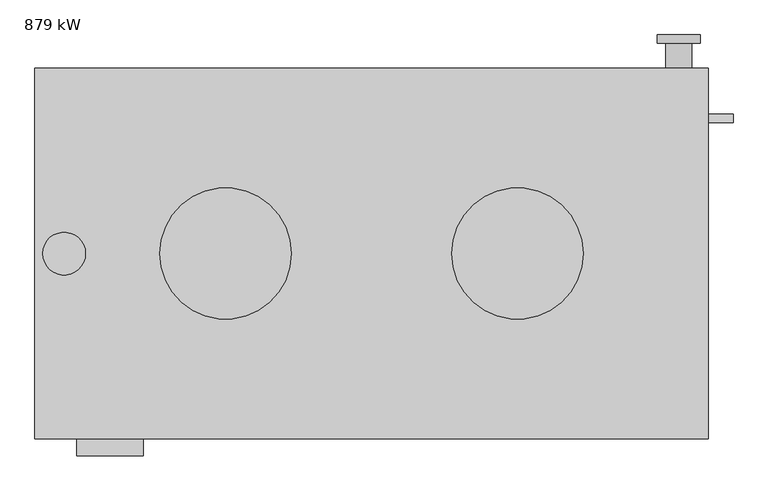
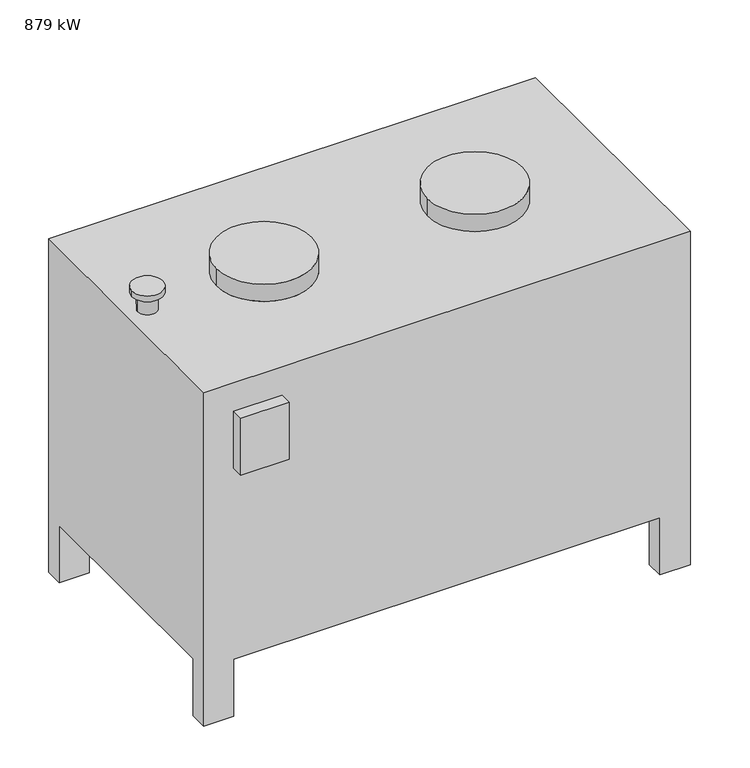
"""IFC4 building model written with IfcOpenShell, lengths in millimetres: proxy geometry, M_Watertube Boiler - 879-6153 kW : 879 kW."""

import ifcopenshell
import ifcopenshell.guid

model = None  # the IFC model being written
_history = None  # IfcOwnerHistory: only IFC2X3 demands one
_inside = {}  # id of a spatial element -> (the spatial element, [elements in it])
_under = {}  # id of a project, library or spatial element -> (it, [spatial elements below it])
_declared = {}  # id of a project -> (the project, [libraries it declares])
_typed = {}  # id of a type object -> (the type object, [elements of that type])
_made_of = {}  # id of a material, layer set ... -> (it, [elements and type objects made of it])


def new_model(schema):
    """Start an empty IFC model of exactly this schema.

    Asked for "IFC4X3", IfcOpenShell would pick the latest addendum, in which some entities
    have other attributes; the version numbers below select the first issue.
    IFC2X3 requires an IfcOwnerHistory on every rooted entity: one is made here for all.
    """
    global model, _history
    if schema == "IFC4X3":
        model = ifcopenshell.file(schema_version=(4, 3, 0, 0))
    else:
        model = ifcopenshell.file(schema=schema)
    _inside.clear()
    _under.clear()
    _declared.clear()
    _typed.clear()
    _made_of.clear()
    _history = None
    if model.schema == "IFC2X3":
        org = make("IfcOrganization", Name="unknown")
        user = make(
            "IfcPersonAndOrganization",
            ThePerson=make("IfcPerson", FamilyName="unknown"),
            TheOrganization=org,
        )
        app = make(
            "IfcApplication",
            ApplicationDeveloper=org,
            Version="unknown",
            ApplicationFullName="unknown",
            ApplicationIdentifier="unknown",
        )
        _history = make(
            "IfcOwnerHistory",
            OwningUser=user,
            OwningApplication=app,
            ChangeAction="ADDED",
            CreationDate=0,
        )
    return model


def make(cls, **values):
    """One entity of the class cls with the attributes given. An attribute that is None is left unset."""
    return model.create_entity(
        cls, **{name: value for name, value in values.items() if value is not None}
    )


def rooted(cls, **values):
    """An entity with a GlobalId (a new one), such as an element, a storey or a relation."""
    return make(cls, GlobalId=ifcopenshell.guid.new(), OwnerHistory=_history, **values)


def si_unit(unit_type, name, prefix=None):
    """IfcSIUnit, for example si_unit("LENGTHUNIT", "METRE", prefix="MILLI")."""
    return make("IfcSIUnit", UnitType=unit_type, Prefix=prefix, Name=name)


def assignment(units):
    """IfcUnitAssignment: the units of a project."""
    return None if units is None else make("IfcUnitAssignment", Units=units)


def point(xyz):
    """IfcCartesianPoint."""
    return None if xyz is None else make("IfcCartesianPoint", Coordinates=xyz)


def direction(xyz):
    """IfcDirection."""
    return None if xyz is None else make("IfcDirection", DirectionRatios=xyz)


def frame(location, z_axis=None, x_axis=None):
    """IfcAxis2Placement3D, a coordinate frame: its origin and axes. An axis left out is left unset."""
    return make(
        "IfcAxis2Placement3D",
        Location=point(location),
        Axis=direction(z_axis),
        RefDirection=direction(x_axis),
    )


def frame_2d(location, x_axis=None):
    """IfcAxis2Placement2D, a coordinate frame in the plane: its origin and x axis."""
    return make(
        "IfcAxis2Placement2D", Location=point(location), RefDirection=direction(x_axis)
    )


def origin():
    """The frame at (0, 0, 0) with its axes left unset."""
    return frame((0.0, 0.0, 0.0))


def place(relative_to, where):
    """IfcLocalPlacement: puts the frame where relative to a parent placement (None: the world)."""
    return make(
        "IfcLocalPlacement", PlacementRelTo=relative_to, RelativePlacement=where
    )


def context(
    kind, dimensions, precision=None, world=None, true_north=None, identifier=None
):
    """IfcGeometricRepresentationContext, for example the 3D "Model" context."""
    return make(
        "IfcGeometricRepresentationContext",
        ContextIdentifier=identifier,
        ContextType=kind,
        CoordinateSpaceDimension=dimensions,
        Precision=precision,
        WorldCoordinateSystem=world,
        TrueNorth=true_north,
    )


def project(units=None, contexts=None):
    """IfcProject with its units and contexts."""
    return rooted(
        "IfcProject",
        Name="project",
        RepresentationContexts=contexts,
        UnitsInContext=assignment(units),
    )


def spatial(cls, under=None, at=None, **own):
    """A site, building, storey or space (cls), placed at a placement, below another one or the project."""
    s = rooted(cls, ObjectPlacement=at, **own)
    if under is not None:
        _under.setdefault(under.id(), (under, []))[1].append(s)
    return s


def circle_curve(where, radius):
    """IfcCircle in the frame where."""
    return make("IfcCircle", Position=where, Radius=radius)


def trimmed(basis, trim1, trim2, sense, master):
    """IfcTrimmedCurve: the piece of a basis curve between two trims."""
    return make(
        "IfcTrimmedCurve",
        BasisCurve=basis,
        Trim1=trim1,
        Trim2=trim2,
        SenseAgreement=sense,
        MasterRepresentation=master,
    )


def segment(curve, same_sense, transition):
    """IfcCompositeCurveSegment."""
    return make(
        "IfcCompositeCurveSegment",
        Transition=transition,
        SameSense=same_sense,
        ParentCurve=curve,
    )


def composite_curve(segments, self_intersect=None):
    """IfcCompositeCurve: segments joined end to end."""
    return make("IfcCompositeCurve", Segments=segments, SelfIntersect=self_intersect)


def outline(outer, holes=None, kind="AREA"):
    """IfcArbitraryClosedProfileDef: a profile drawn as a closed curve; with holes, ...WithVoids."""
    if holes is None:
        return make("IfcArbitraryClosedProfileDef", ProfileType=kind, OuterCurve=outer)
    return make(
        "IfcArbitraryProfileDefWithVoids",
        ProfileType=kind,
        OuterCurve=outer,
        InnerCurves=holes,
    )


def extrude(swept, where, along, depth):
    """IfcExtrudedAreaSolid: the profile swept, set in the frame where, extruded along a direction by depth."""
    return make(
        "IfcExtrudedAreaSolid",
        SweptArea=swept,
        Position=where,
        ExtrudedDirection=direction(along),
        Depth=depth,
    )


def shape(context_of_items, identifier, shape_type, items):
    """IfcShapeRepresentation: the items that make up one representation, for example the "Body"."""
    return make(
        "IfcShapeRepresentation",
        ContextOfItems=context_of_items,
        RepresentationIdentifier=identifier,
        RepresentationType=shape_type,
        Items=items,
    )


def source(mapping_origin, context_of_items, identifier, shape_type, items):
    """IfcRepresentationMap: a shape defined once, which mapped items show again and again."""
    return make(
        "IfcRepresentationMap",
        MappingOrigin=mapping_origin,
        MappedRepresentation=shape(context_of_items, identifier, shape_type, items),
    )


def transform(
    local_origin,
    x_axis=None,
    y_axis=None,
    z_axis=None,
    scale=None,
    scale2=None,
    scale3=None,
    uniform=True,
):
    """IfcCartesianTransformationOperator3D, or its non-uniform kind. x_axis, y_axis, z_axis: its Axis1, 2, 3."""
    if uniform:
        return make(
            "IfcCartesianTransformationOperator3D",
            Axis1=direction(x_axis),
            Axis2=direction(y_axis),
            LocalOrigin=point(local_origin),
            Scale=scale,
            Axis3=direction(z_axis),
        )
    return make(
        "IfcCartesianTransformationOperator3DnonUniform",
        Axis1=direction(x_axis),
        Axis2=direction(y_axis),
        LocalOrigin=point(local_origin),
        Scale=scale,
        Axis3=direction(z_axis),
        Scale2=scale2,
        Scale3=scale3,
    )


def mapped(mapping_source, mapping_target):
    """IfcMappedItem: shows the shape of a source again, moved by a transform."""
    return make(
        "IfcMappedItem", MappingSource=mapping_source, MappingTarget=mapping_target
    )


def made_of(thing, what):
    """Note that an element or type object is made of a material, layer set ...; save() writes the relation."""
    if what is not None:
        _made_of.setdefault(what.id(), (what, []))[1].append(thing)
    return thing


def element(
    cls,
    number,
    at=None,
    inside=None,
    cuts=None,
    type_object=None,
    material=None,
    context=None,
    identifier="Body",
    shape_type=None,
    held_by="IfcProductDefinitionShape",
    body=None,
    shapes=None,
    **own,
):
    """One element of the class cls, such as IfcWall. Its Tag is "e" and its number.

    at: its placement. inside: the storey or other place that contains it. cuts: it is an
    opening in that element (IfcRelVoidsElement). A single representation is given by context,
    identifier, shape_type and body (its items); several are given by shapes. held_by: the class
    of the entity that holds the representations. save() writes the other relations.
    """
    e = rooted(cls, Tag="e%d" % number, ObjectPlacement=at, **own)
    if body is not None:
        shapes = [shape(context, identifier, shape_type, body)]
    if shapes is not None:
        e.Representation = make(held_by, Representations=shapes)
    if inside is not None:
        _inside.setdefault(inside.id(), (inside, []))[1].append(e)
    if cuts is not None:
        rooted(
            "IfcRelVoidsElement", RelatingBuildingElement=cuts, RelatedOpeningElement=e
        )
    if type_object is not None:
        _typed.setdefault(type_object.id(), (type_object, []))[1].append(e)
    return made_of(e, material)


def aggregate(whole, parts):
    """IfcRelAggregates: a whole, such as a stair, and the parts it consists of."""
    return rooted("IfcRelAggregates", RelatingObject=whole, RelatedObjects=parts)


def save(model, path):
    """Write the relations noted so far, then the file.

    IfcRelAggregates (storeys below a building ...), IfcRelContainedInSpatialStructure (elements
    in a storey), IfcRelDefinesByType, IfcRelAssociatesMaterial and IfcRelDeclares: one each for
    every whole, place, type object, material and project.
    """
    for whole, parts in _under.values():
        aggregate(whole, parts)
    for where, things in _inside.values():
        rooted(
            "IfcRelContainedInSpatialStructure",
            RelatedElements=things,
            RelatingStructure=where,
        )
    for kind, things in _typed.values():
        rooted("IfcRelDefinesByType", RelatedObjects=things, RelatingType=kind)
    for what, things in _made_of.values():
        rooted("IfcRelAssociatesMaterial", RelatedObjects=things, RelatingMaterial=what)
    for by, libraries in _declared.values():
        rooted("IfcRelDeclares", RelatingContext=by, RelatedDefinitions=libraries)
    model.write(path)


def plane_surface(at):
    """IfcPlane: the flat surface through the origin of the frame at, square to its z axis."""
    return make("IfcPlane", Position=at)


def cylinder_surface(at, radius):
    """IfcCylindricalSurface: all points at the distance radius from the z axis of the frame at."""
    return make("IfcCylindricalSurface", Position=at, Radius=radius)


def advanced_brep(points, edges, surfaces, faces):
    """IfcAdvancedBrep: a solid bounded by faces that lie on surfaces and meet in shared edges.

    An edge is (start, end): straight between two places in points (the first is 0);
    or (start, end, curve); or (start, end, curve, False) where it runs against its curve.
    A face is (place in surfaces, loops), or (place, loops, False) where it looks against
    its surface's normal. A loop lists edges by number (the first is 1), with a minus sign
    where the edge is run from its end to its start. The first loop is the outer one.
    """
    corners = [point(p) for p in points]
    vertices = [make("IfcVertexPoint", VertexGeometry=c) for c in corners]
    made = []
    for start, end, *more in edges:
        made.append(
            make(
                "IfcEdgeCurve",
                EdgeStart=vertices[start],
                EdgeEnd=vertices[end],
                EdgeGeometry=more[0] if more else make("IfcPolyline", Points=[corners[start], corners[end]]),
                SameSense=more[1] if len(more) > 1 else True,
            )
        )
    hull = []
    for where, loops, *sense in faces:
        bounds = []
        for j, loop in enumerate(loops):
            ring = [make("IfcOrientedEdge", EdgeElement=made[abs(k) - 1], Orientation=k > 0) for k in loop]
            bounds.append(
                make(
                    "IfcFaceOuterBound" if j == 0 else "IfcFaceBound",
                    Bound=make("IfcEdgeLoop", EdgeList=ring),
                    Orientation=True,
                )
            )
        hull.append(make("IfcAdvancedFace", Bounds=bounds, FaceSurface=surfaces[where], SameSense=sense[0] if sense else True))
    return make("IfcAdvancedBrep", Outer=make("IfcClosedShell", CfsFaces=hull))


def proxy_879_kw_a7649213(model_context):
    return source(origin(), model_context, "Body", "SolidModel", [
        extrude(outline(composite_curve([segment(trimmed(circle_curve(frame_2d((826.0, 1961.0)), 40.0), [point((826.0, 1921.0))], [point((826.0, 2001.0))], False, "CARTESIAN"), True, "CONTINUOUS"), segment(trimmed(circle_curve(frame_2d((826.0, 1961.0)), 40.0), [point((826.0, 2001.0))], [point((826.0, 1921.0))], False, "CARTESIAN"), True, "CONTINUOUS")], self_intersect=False)), frame((0.0, 1130.0, 0.0), z_axis=(0.0, 1.0, 0.0), x_axis=(0.0, 0.0, 1.0)), (0.0, 0.0, 1.0), 76.2),
        extrude(outline(composite_curve([segment(trimmed(circle_curve(frame_2d((826.0, 1961.0)), 65.0), [point((826.0, 1896.0))], [point((826.0, 2026.0))], False, "CARTESIAN"), True, "CONTINUOUS"), segment(trimmed(circle_curve(frame_2d((826.0, 1961.0)), 65.0), [point((826.0, 2026.0))], [point((826.0, 1896.0))], False, "CARTESIAN"), True, "CONTINUOUS")], self_intersect=False)), frame((0.0, 1206.5, 0.0), z_axis=(0.0, 1.0, 0.0), x_axis=(0.0, 0.0, 1.0)), (0.0, 0.0, 1.0), 25.1),
        extrude(outline(composite_curve([segment(trimmed(circle_curve(frame_2d((977.6, 508.0)), 12.7), [point((964.9, 508.0))], [point((990.3, 508.0))], False, "CARTESIAN"), True, "CONTINUOUS"), segment(trimmed(circle_curve(frame_2d((977.6, 508.0)), 12.7), [point((990.3, 508.0))], [point((964.9, 508.0))], False, "CARTESIAN"), True, "CONTINUOUS")], self_intersect=False)), frame((2050.0, 0.0, 0.0), z_axis=(1.0, 0.0, 0.0), x_axis=(0.0, 1.0, 0.0)), (0.0, 0.0, 1.0), 76.2),
        extrude(outline(composite_curve([segment(trimmed(circle_curve(frame_2d((1796.0, 203.2)), 25.0), [point((1771.0, 203.2))], [point((1821.0, 203.2))], False, "CARTESIAN"), True, "CONTINUOUS"), segment(trimmed(circle_curve(frame_2d((1796.0, 203.2)), 25.0), [point((1821.0, 203.2))], [point((1771.0, 203.2))], False, "CARTESIAN"), True, "CONTINUOUS")], self_intersect=False)), frame((0.0, 0.0, 177.8), z_axis=(0.0, 0.0, 1.0), x_axis=(1.0, 0.0, 0.0)), (0.0, 0.0, 1.0), 76.2),
        advanced_brep(
        [(1923.0, 0.0, 254.0), (1923.0, 0.0, 0.0), (2050.0, 0.0, 0.0), (2050.0, 0.0, 1485.0), (0.0, 0.0, 1485.0), (0.0, 0.0, 0.0), (127.0, 0.0, 0.0), (127.0, 0.0, 254.0), (127.0, 0.0, 1358.0), (330.2, 0.0, 1358.0), (330.2, 0.0, 1104.0), (127.0, 0.0, 1104.0), (2050.0, 76.2, 254.0), (2050.0, 76.2, 0.0), (1923.0, 76.2, 0.0), (1923.0, 76.2, 254.0), (2050.0, 1053.8, 254.0), (2050.0, 1053.8, 0.0), (2050.0, 1130.0, 0.0), (2050.0, 1130.0, 1485.0), (1923.0, 1053.8, 254.0), (1923.0, 1053.8, 0.0), (1923.0, 1130.0, 0.0), (1923.0, 1130.0, 254.0), (127.0, 1130.0, 254.0), (127.0, 1130.0, 0.0), (0.0, 1130.0, 0.0), (0.0, 1130.0, 1485.0), (129.0, 565.0, 1485.0), (49.0, 565.0, 1485.0), (780.5, 565.0, 1485.0), (380.5, 565.0, 1485.0), (1669.5, 565.0, 1485.0), (1269.5, 565.0, 1485.0), (127.0, 76.2, 254.0), (0.0, 76.2, 254.0), (0.0, 1053.8, 254.0), (127.0, 1053.8, 254.0), (0.0, 1053.8, 0.0), (0.0, 76.2, 0.0), (49.0, 565.0, 1561.2), (129.0, 565.0, 1561.2), (24.0, 565.0, 1586.6), (154.0, 565.0, 1586.6), (24.0, 565.0, 1561.2), (154.0, 565.0, 1561.2), (380.5, 565.0, 1561.2), (780.5, 565.0, 1561.2), (1269.5, 565.0, 1561.2), (1669.5, 565.0, 1561.2), (330.2, -50.8, 1358.0), (127.0, -50.8, 1358.0), (127.0, -50.8, 1104.0), (330.2, -50.8, 1104.0), (127.0, 76.2, 0.0), (127.0, 1053.8, 0.0)],
        [
            (0, 1),
            (1, 2),
            (2, 3),
            (3, 4),
            (4, 5),
            (5, 6),
            (6, 7),
            (7, 0),
            (8, 9),
            (9, 10),
            (10, 11),
            (11, 8),
            (12, 13),
            (13, 14),
            (14, 15),
            (15, 12),
            (0, 15),
            (14, 1),
            (13, 2),
            (12, 16),
            (16, 17),
            (17, 18),
            (18, 19),
            (19, 3),
            (20, 21),
            (21, 17),
            (16, 20),
            (18, 22),
            (22, 23),
            (23, 24),
            (24, 25),
            (25, 26),
            (26, 27),
            (27, 19),
            (20, 23),
            (22, 21),
            (27, 4),
            (28, 29, circle_curve(frame((89.0, 565.0, 1485.0), z_axis=(0.0, 0.0, -1.0), x_axis=(1.0, 0.0, 0.0)), 40.0)),
            (29, 28, circle_curve(frame((89.0, 565.0, 1485.0), z_axis=(0.0, 0.0, -1.0), x_axis=(1.0, 0.0, 0.0)), 40.0)),
            (30, 31, circle_curve(frame((580.5, 565.0, 1485.0), z_axis=(0.0, 0.0, -1.0), x_axis=(1.0, 0.0, 0.0)), 200.0)),
            (31, 30, circle_curve(frame((580.5, 565.0, 1485.0), z_axis=(0.0, 0.0, -1.0), x_axis=(1.0, 0.0, 0.0)), 200.0)),
            (32, 33, circle_curve(frame((1469.5, 565.0, 1485.0), z_axis=(0.0, 0.0, -1.0), x_axis=(1.0, 0.0, 0.0)), 200.0)),
            (33, 32, circle_curve(frame((1469.5, 565.0, 1485.0), z_axis=(0.0, 0.0, -1.0), x_axis=(1.0, 0.0, 0.0)), 200.0)),
            (7, 34),
            (34, 35),
            (35, 36),
            (36, 37),
            (37, 24),
            (26, 38),
            (38, 36),
            (35, 39),
            (39, 5),
            (40, 29),
            (28, 41),
            (41, 40, circle_curve(frame((89.0, 565.0, 1561.2), z_axis=(0.0, 0.0, -1.0), x_axis=(1.0, 0.0, 0.0)), 40.0)),
            (40, 41, circle_curve(frame((89.0, 565.0, 1561.2), z_axis=(0.0, 0.0, -1.0), x_axis=(1.0, 0.0, 0.0)), 40.0)),
            (42, 43, circle_curve(frame((89.0, 565.0, 1586.6), z_axis=(0.0, 0.0, 1.0), x_axis=(1.0, 0.0, 0.0)), 65.0)),
            (43, 42, circle_curve(frame((89.0, 565.0, 1586.6), z_axis=(0.0, 0.0, 1.0), x_axis=(1.0, 0.0, 0.0)), 65.0)),
            (44, 45, circle_curve(frame((89.0, 565.0, 1561.2), z_axis=(0.0, 0.0, -1.0), x_axis=(1.0, 0.0, 0.0)), 65.0)),
            (45, 44, circle_curve(frame((89.0, 565.0, 1561.2), z_axis=(0.0, 0.0, -1.0), x_axis=(1.0, 0.0, 0.0)), 65.0)),
            (42, 44),
            (45, 43),
            (46, 47, circle_curve(frame((580.5, 565.0, 1561.2), z_axis=(0.0, 0.0, 1.0), x_axis=(1.0, 0.0, 0.0)), 200.0)),
            (47, 46, circle_curve(frame((580.5, 565.0, 1561.2), z_axis=(0.0, 0.0, 1.0), x_axis=(1.0, 0.0, 0.0)), 200.0)),
            (48, 49, circle_curve(frame((1469.5, 565.0, 1561.2), z_axis=(0.0, 0.0, 1.0), x_axis=(1.0, 0.0, 0.0)), 200.0)),
            (49, 48, circle_curve(frame((1469.5, 565.0, 1561.2), z_axis=(0.0, 0.0, 1.0), x_axis=(1.0, 0.0, 0.0)), 200.0)),
            (46, 31),
            (30, 47),
            (48, 33),
            (32, 49),
            (50, 51),
            (51, 52),
            (52, 53),
            (53, 50),
            (50, 9),
            (8, 51),
            (11, 52),
            (10, 53),
            (34, 54),
            (54, 39),
            (54, 6),
            (38, 55),
            (55, 37),
            (25, 55),
        ],
        [
            plane_surface(frame((1923.0, 0.0, 254.0), z_axis=(0.0, -1.0, 0.0), x_axis=(0.0, 0.0, -1.0))),
            plane_surface(frame((1923.0, 76.2, 254.0), z_axis=(0.0, 1.0, 0.0), x_axis=(0.0, 0.0, 1.0))),
            plane_surface(frame((1923.0, 0.0, 254.0), z_axis=(-1.0, 0.0, 0.0), x_axis=(0.0, 1.0, 0.0))),
            plane_surface(frame((1923.0, 0.0, 0.0), z_axis=(0.0, 0.0, -1.0), x_axis=(0.0, 1.0, 0.0))),
            plane_surface(frame((2050.0, 0.0, 0.0), z_axis=(1.0, 0.0, 0.0), x_axis=(0.0, 1.0, 0.0))),
            plane_surface(frame((1923.0, 1053.8, 254.0), z_axis=(0.0, -1.0, 0.0), x_axis=(0.0, 0.0, -1.0))),
            plane_surface(frame((1923.0, 1130.0, 254.0), z_axis=(0.0, 1.0, 0.0), x_axis=(0.0, 0.0, 1.0))),
            plane_surface(frame((1923.0, 1053.8, 254.0), z_axis=(-1.0, 0.0, 0.0), x_axis=(0.0, 1.0, 0.0))),
            plane_surface(frame((1923.0, 1053.8, 0.0), z_axis=(0.0, 0.0, -1.0), x_axis=(0.0, 1.0, 0.0))),
            plane_surface(frame((0.0, 1130.0, 1485.0), z_axis=(0.0, 0.0, 1.0), x_axis=(-1.0, 0.0, 0.0))),
            plane_surface(frame((0.0, 1130.0, 254.0), z_axis=(0.0, 0.0, -1.0), x_axis=(1.0, 0.0, 0.0))),
            plane_surface(frame((0.0, 1130.0, 1485.0), z_axis=(-1.0, 0.0, 0.0), x_axis=(0.0, 0.0, -1.0))),
            cylinder_surface(frame((89.0, 565.0, 1485.0), z_axis=(0.0, 0.0, 1.0), x_axis=(1.0, 0.0, 0.0)), 40.0),
            plane_surface(frame((154.0, 565.0, 1586.6), z_axis=(0.0, 0.0, 1.0), x_axis=(0.0, 1.0, 0.0))),
            plane_surface(frame((154.0, 565.0, 1561.2), z_axis=(0.0, 0.0, -1.0), x_axis=(0.0, -1.0, 0.0))),
            cylinder_surface(frame((89.0, 565.0, 1561.2), z_axis=(0.0, 0.0, 1.0), x_axis=(1.0, 0.0, 0.0)), 65.0),
            plane_surface(frame((780.5, 565.0, 1561.2), z_axis=(0.0, 0.0, 1.0), x_axis=(0.0, 1.0, 0.0))),
            cylinder_surface(frame((580.5, 565.0, 1485.0), z_axis=(0.0, 0.0, 1.0), x_axis=(1.0, 0.0, 0.0)), 200.0),
            cylinder_surface(frame((1469.5, 565.0, 0.0), z_axis=(0.0, 0.0, 1.0), x_axis=(1.0, 0.0, 0.0)), 200.0),
            plane_surface(frame((127.0, -50.8, 1358.0), z_axis=(0.0, -1.0, 0.0), x_axis=(-1.0, 0.0, 0.0))),
            plane_surface(frame((330.2, -50.8, 1358.0), z_axis=(0.0, 0.0, 1.0), x_axis=(0.0, 1.0, 0.0))),
            plane_surface(frame((127.0, -50.8, 1358.0), z_axis=(-1.0, 0.0, 0.0), x_axis=(0.0, 1.0, 0.0))),
            plane_surface(frame((127.0, -50.8, 1104.0), z_axis=(0.0, 0.0, -1.0), x_axis=(0.0, 1.0, 0.0))),
            plane_surface(frame((330.2, -50.8, 1104.0), z_axis=(1.0, 0.0, 0.0), x_axis=(0.0, 1.0, 0.0))),
            plane_surface(frame((127.0, 76.2, 0.0), z_axis=(0.0, 1.0, 0.0), x_axis=(-1.0, 0.0, 0.0))),
            plane_surface(frame((0.0, 0.0, 0.0), z_axis=(0.0, 0.0, -1.0), x_axis=(0.0, 1.0, 0.0))),
            plane_surface(frame((127.0, 0.0, 0.0), z_axis=(1.0, 0.0, 0.0), x_axis=(0.0, 1.0, 0.0))),
            plane_surface(frame((0.0, 1053.8, 173.9475615), z_axis=(0.0, -1.0, 0.0), x_axis=(0.0, 0.0, -1.0))),
            plane_surface(frame((0.0, 1053.8, 0.0), z_axis=(0.0, 0.0, -1.0), x_axis=(0.0, 1.0, 0.0))),
            plane_surface(frame((127.0, 1053.8, 0.0), z_axis=(1.0, 0.0, 0.0), x_axis=(0.0, 1.0, 0.0))),
        ],
        [
            (0, [[1, 2, 3, 4, 5, 6, 7, 8], [9, 10, 11, 12]]),
            (1, [[13, 14, 15, 16]]),
            (2, [[-1, 17, -15, 18]]),
            (3, [[-2, -18, -14, 19]]),
            (4, [[-13, 20, 21, 22, 23, 24, -3, -19]]),
            (5, [[25, 26, -21, 27]]),
            (6, [[28, 29, 30, 31, 32, 33, 34, -23]]),
            (7, [[-25, 35, -29, 36]]),
            (8, [[-26, -36, -28, -22]]),
            (9, [[-34, 37, -4, -24], [38, 39], [40, 41], [42, 43]]),
            (10, [[-20, -16, -17, -8, 44, 45, 46, 47, 48, -30, -35, -27]]),
            (11, [[-37, -33, 49, 50, -46, 51, 52, -5]]),
            (12, [[53, -38, 54, 55]]),
            (12, [[-53, 56, -54, -39]]),
            (13, [[57, 58]]),
            (14, [[59, 60], [-55, -56]]),
            (15, [[-57, 61, -60, 62]]),
            (15, [[-58, -62, -59, -61]]),
            (16, [[63, 64]]),
            (16, [[65, 66]]),
            (17, [[-63, 67, -40, 68]]),
            (17, [[-64, -68, -41, -67]]),
            (18, [[-65, 69, -42, 70]]),
            (18, [[-66, -70, -43, -69]]),
            (19, [[71, 72, 73, 74]]),
            (20, [[-71, 75, -9, 76]]),
            (21, [[-72, -76, -12, 77]]),
            (22, [[-73, -77, -11, 78]]),
            (23, [[-74, -78, -10, -75]]),
            (24, [[-51, -45, 79, 80]]),
            (25, [[-6, -52, -80, 81]]),
            (26, [[-7, -81, -79, -44]]),
            (27, [[-50, 82, 83, -47]]),
            (28, [[-82, -49, -32, 84]]),
            (29, [[-83, -84, -31, -48]]),
        ],
    ),
        extrude(outline(composite_curve([segment(trimmed(circle_curve(frame_2d((977.6, 508.0)), 12.7), [point((964.9, 508.0))], [point((990.3, 508.0))], False, "CARTESIAN"), True, "CONTINUOUS"), segment(trimmed(circle_curve(frame_2d((977.6, 508.0)), 12.7), [point((990.3, 508.0))], [point((964.9, 508.0))], False, "CARTESIAN"), True, "CONTINUOUS")], self_intersect=False)), frame((2050.0, 0.0, 0.0), z_axis=(1.0, 0.0, 0.0), x_axis=(0.0, 1.0, 0.0)), (0.0, 0.0, 1.0), 76.2),
        extrude(outline(composite_curve([segment(trimmed(circle_curve(frame_2d((826.0, 1961.0)), 40.0), [point((826.0, 1921.0))], [point((826.0, 2001.0))], False, "CARTESIAN"), True, "CONTINUOUS"), segment(trimmed(circle_curve(frame_2d((826.0, 1961.0)), 40.0), [point((826.0, 2001.0))], [point((826.0, 1921.0))], False, "CARTESIAN"), True, "CONTINUOUS")], self_intersect=False)), frame((0.0, 1130.0, 0.0), z_axis=(0.0, 1.0, 0.0), x_axis=(0.0, 0.0, 1.0)), (0.0, 0.0, 1.0), 76.2),
        extrude(outline(composite_curve([segment(trimmed(circle_curve(frame_2d((826.0, 1961.0)), 65.0), [point((826.0, 1896.0))], [point((826.0, 2026.0))], False, "CARTESIAN"), True, "CONTINUOUS"), segment(trimmed(circle_curve(frame_2d((826.0, 1961.0)), 65.0), [point((826.0, 2026.0))], [point((826.0, 1896.0))], False, "CARTESIAN"), True, "CONTINUOUS")], self_intersect=False)), frame((0.0, 1206.2, 0.0), z_axis=(0.0, 1.0, 0.0), x_axis=(0.0, 0.0, 1.0)), (0.0, 0.0, 1.0), 25.4),
    ])


if __name__ == "__main__":
    model = new_model("IFC4")
    model_context = context("Model", 3, world=origin())
    ifc_project = project(units=[si_unit("LENGTHUNIT", "METRE", prefix="MILLI")], contexts=[model_context])
    site = spatial("IfcSite", under=ifc_project)
    building = spatial("IfcBuilding", under=site)
    placement = place(None, origin())
    proxy_879_kw_shape = proxy_879_kw_a7649213(model_context)
    element("IfcBuildingElementProxy", 1, Name="M_Watertube Boiler - 879-6153 kW : 879 kW", ObjectType="M_Watertube Boiler - 879-6153 kW : 879 kW", at=placement, inside=building, context=model_context, shape_type="MappedRepresentation", body=[
        mapped(proxy_879_kw_shape, transform((0.0, 0.0, 0.0), x_axis=(1.0, 0.0, 0.0), y_axis=(0.0, 1.0, 0.0), z_axis=(0.0, 0.0, 1.0))),
    ])
    save(model, "model.ifc")

# Revit data of these elements
# Type "M_Watertube Boiler - 879-6153 kW : 879 kW"
#   Model = "096967565434gdewtg"
#   Manufacturer = "Boilers Inc"
#   Description = "Boiler"
#   COBie.Type.CreatedBy = "design@eagle.com"
#   COBie.Type.CreatedOn = "2016-09-13T05:47:35"
#   COBie.Type.Name = "Mechanical Equipment_M_Watertube Boiler - 879-6153 kW_879 kW"
#   COBie.Type.Category = "23-75 10 11 14 34 : Steel Water-Tube Boilers"
#   COBie.Type.Description = "Boiler"
#   COBie.Type.Manufacturer = "Boilers Inc"
#   COBie.Type.ModelNumber = "096967565434gdewtg"
#   COBie.Type.ReplacementCost = 0
#   Water Volume [instance default] = 4.22 m³
#   Water Pressure Drop [instance default] = 11700.0 Pa
#   Water Flow [instance default] = 15.8 L/s
#   Voltage = 120 V
#   Vent Radius = 200 mm
#   Vent Duct Length = 889 mm
#   Vent Diameter = 400 mm
#   Radius 2 = 65 mm
#   Radius 1 = 65 mm
#   Pipe Length 2 = 89 mm
#   Pipe Length 1 = 89 mm
#   Pipe Height 1 = 826 mm
#   Output Heat [instance default] = 730000 W
#   Input Heat [instance default] = 879000 W
#   Hot Water Radius = 40 mm
#   Hot Water Diameter = 80 mm
#   Heating Surface = 35.5 m²
#   Gas Radius = 25 mm
#   Gas Flow [instance default] = 0.0 L/s
#   Gas Diameter = 50 mm
#   Exhaust Air Flow [instance default] = 0.0 L/s
#   Cold Water Radius = 40 mm
#   Cold Water Diameter = 80 mm
#   Boiler Width = 1130 mm
#   Boiler Length = 2050 mm
#   Boiler Height = 1485 mm
#   BHP [instance default] = 74.4
#   Apparent Load = 480 VA
#   COBie.Type = yes
#   Number of Poles = 1
#   Boiler Material = none
